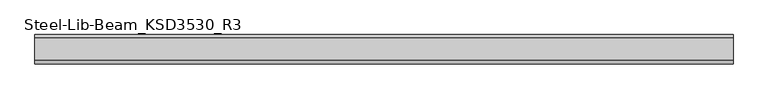
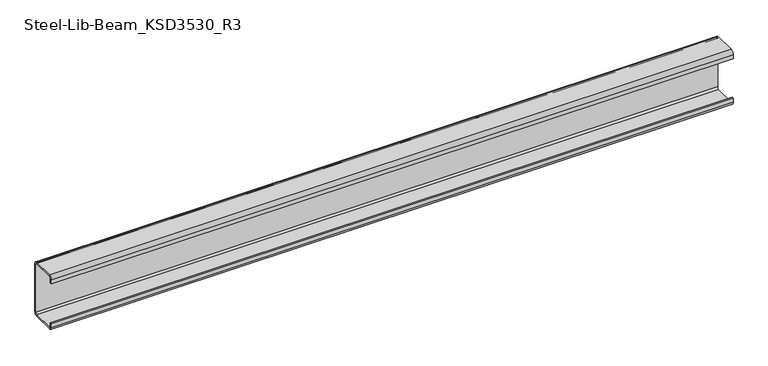
"""IFC4 building model written with IfcOpenShell, lengths in millimetres: beam geometry, Steel-Lib-Beam_KSD3530_R3 : BMS291_C-150×75x20x4.5."""

import ifcopenshell
import ifcopenshell.guid

model = None  # the IFC model being written
_history = None  # IfcOwnerHistory: only IFC2X3 demands one
_inside = {}  # id of a spatial element -> (the spatial element, [elements in it])
_under = {}  # id of a project, library or spatial element -> (it, [spatial elements below it])
_declared = {}  # id of a project -> (the project, [libraries it declares])
_typed = {}  # id of a type object -> (the type object, [elements of that type])
_made_of = {}  # id of a material, layer set ... -> (it, [elements and type objects made of it])


def new_model(schema):
    """Start an empty IFC model of exactly this schema.

    Asked for "IFC4X3", IfcOpenShell would pick the latest addendum, in which some entities
    have other attributes; the version numbers below select the first issue.
    IFC2X3 requires an IfcOwnerHistory on every rooted entity: one is made here for all.
    """
    global model, _history
    if schema == "IFC4X3":
        model = ifcopenshell.file(schema_version=(4, 3, 0, 0))
    else:
        model = ifcopenshell.file(schema=schema)
    _inside.clear()
    _under.clear()
    _declared.clear()
    _typed.clear()
    _made_of.clear()
    _history = None
    if model.schema == "IFC2X3":
        org = make("IfcOrganization", Name="unknown")
        user = make(
            "IfcPersonAndOrganization",
            ThePerson=make("IfcPerson", FamilyName="unknown"),
            TheOrganization=org,
        )
        app = make(
            "IfcApplication",
            ApplicationDeveloper=org,
            Version="unknown",
            ApplicationFullName="unknown",
            ApplicationIdentifier="unknown",
        )
        _history = make(
            "IfcOwnerHistory",
            OwningUser=user,
            OwningApplication=app,
            ChangeAction="ADDED",
            CreationDate=0,
        )
    return model


def make(cls, **values):
    """One entity of the class cls with the attributes given. An attribute that is None is left unset."""
    return model.create_entity(
        cls, **{name: value for name, value in values.items() if value is not None}
    )


def rooted(cls, **values):
    """An entity with a GlobalId (a new one), such as an element, a storey or a relation."""
    return make(cls, GlobalId=ifcopenshell.guid.new(), OwnerHistory=_history, **values)


def si_unit(unit_type, name, prefix=None):
    """IfcSIUnit, for example si_unit("LENGTHUNIT", "METRE", prefix="MILLI")."""
    return make("IfcSIUnit", UnitType=unit_type, Prefix=prefix, Name=name)


def assignment(units):
    """IfcUnitAssignment: the units of a project."""
    return None if units is None else make("IfcUnitAssignment", Units=units)


def point(xyz):
    """IfcCartesianPoint."""
    return None if xyz is None else make("IfcCartesianPoint", Coordinates=xyz)


def direction(xyz):
    """IfcDirection."""
    return None if xyz is None else make("IfcDirection", DirectionRatios=xyz)


def frame(location, z_axis=None, x_axis=None):
    """IfcAxis2Placement3D, a coordinate frame: its origin and axes. An axis left out is left unset."""
    return make(
        "IfcAxis2Placement3D",
        Location=point(location),
        Axis=direction(z_axis),
        RefDirection=direction(x_axis),
    )


def frame_2d(location, x_axis=None):
    """IfcAxis2Placement2D, a coordinate frame in the plane: its origin and x axis."""
    return make(
        "IfcAxis2Placement2D", Location=point(location), RefDirection=direction(x_axis)
    )


def origin():
    """The frame at (0, 0, 0) with its axes left unset."""
    return frame((0.0, 0.0, 0.0))


def place(relative_to, where):
    """IfcLocalPlacement: puts the frame where relative to a parent placement (None: the world)."""
    return make(
        "IfcLocalPlacement", PlacementRelTo=relative_to, RelativePlacement=where
    )


def context(
    kind, dimensions, precision=None, world=None, true_north=None, identifier=None
):
    """IfcGeometricRepresentationContext, for example the 3D "Model" context."""
    return make(
        "IfcGeometricRepresentationContext",
        ContextIdentifier=identifier,
        ContextType=kind,
        CoordinateSpaceDimension=dimensions,
        Precision=precision,
        WorldCoordinateSystem=world,
        TrueNorth=true_north,
    )


def project(units=None, contexts=None):
    """IfcProject with its units and contexts."""
    return rooted(
        "IfcProject",
        Name="project",
        RepresentationContexts=contexts,
        UnitsInContext=assignment(units),
    )


def spatial(cls, under=None, at=None, **own):
    """A site, building, storey or space (cls), placed at a placement, below another one or the project."""
    s = rooted(cls, ObjectPlacement=at, **own)
    if under is not None:
        _under.setdefault(under.id(), (under, []))[1].append(s)
    return s


def polyline(points):
    """IfcPolyline through the points."""
    return make("IfcPolyline", Points=[point(p) for p in points])


def circle_curve(where, radius):
    """IfcCircle in the frame where."""
    return make("IfcCircle", Position=where, Radius=radius)


def trimmed(basis, trim1, trim2, sense, master):
    """IfcTrimmedCurve: the piece of a basis curve between two trims."""
    return make(
        "IfcTrimmedCurve",
        BasisCurve=basis,
        Trim1=trim1,
        Trim2=trim2,
        SenseAgreement=sense,
        MasterRepresentation=master,
    )


def segment(curve, same_sense, transition):
    """IfcCompositeCurveSegment."""
    return make(
        "IfcCompositeCurveSegment",
        Transition=transition,
        SameSense=same_sense,
        ParentCurve=curve,
    )


def composite_curve(segments, self_intersect=None):
    """IfcCompositeCurve: segments joined end to end."""
    return make("IfcCompositeCurve", Segments=segments, SelfIntersect=self_intersect)


def outline(outer, holes=None, kind="AREA"):
    """IfcArbitraryClosedProfileDef: a profile drawn as a closed curve; with holes, ...WithVoids."""
    if holes is None:
        return make("IfcArbitraryClosedProfileDef", ProfileType=kind, OuterCurve=outer)
    return make(
        "IfcArbitraryProfileDefWithVoids",
        ProfileType=kind,
        OuterCurve=outer,
        InnerCurves=holes,
    )


def extrude(swept, where, along, depth):
    """IfcExtrudedAreaSolid: the profile swept, set in the frame where, extruded along a direction by depth."""
    return make(
        "IfcExtrudedAreaSolid",
        SweptArea=swept,
        Position=where,
        ExtrudedDirection=direction(along),
        Depth=depth,
    )


def shape(context_of_items, identifier, shape_type, items):
    """IfcShapeRepresentation: the items that make up one representation, for example the "Body"."""
    return make(
        "IfcShapeRepresentation",
        ContextOfItems=context_of_items,
        RepresentationIdentifier=identifier,
        RepresentationType=shape_type,
        Items=items,
    )


def source(mapping_origin, context_of_items, identifier, shape_type, items):
    """IfcRepresentationMap: a shape defined once, which mapped items show again and again."""
    return make(
        "IfcRepresentationMap",
        MappingOrigin=mapping_origin,
        MappedRepresentation=shape(context_of_items, identifier, shape_type, items),
    )


def transform(
    local_origin,
    x_axis=None,
    y_axis=None,
    z_axis=None,
    scale=None,
    scale2=None,
    scale3=None,
    uniform=True,
):
    """IfcCartesianTransformationOperator3D, or its non-uniform kind. x_axis, y_axis, z_axis: its Axis1, 2, 3."""
    if uniform:
        return make(
            "IfcCartesianTransformationOperator3D",
            Axis1=direction(x_axis),
            Axis2=direction(y_axis),
            LocalOrigin=point(local_origin),
            Scale=scale,
            Axis3=direction(z_axis),
        )
    return make(
        "IfcCartesianTransformationOperator3DnonUniform",
        Axis1=direction(x_axis),
        Axis2=direction(y_axis),
        LocalOrigin=point(local_origin),
        Scale=scale,
        Axis3=direction(z_axis),
        Scale2=scale2,
        Scale3=scale3,
    )


def mapped(mapping_source, mapping_target):
    """IfcMappedItem: shows the shape of a source again, moved by a transform."""
    return make(
        "IfcMappedItem", MappingSource=mapping_source, MappingTarget=mapping_target
    )


def made_of(thing, what):
    """Note that an element or type object is made of a material, layer set ...; save() writes the relation."""
    if what is not None:
        _made_of.setdefault(what.id(), (what, []))[1].append(thing)
    return thing


def element(
    cls,
    number,
    at=None,
    inside=None,
    cuts=None,
    type_object=None,
    material=None,
    context=None,
    identifier="Body",
    shape_type=None,
    held_by="IfcProductDefinitionShape",
    body=None,
    shapes=None,
    **own,
):
    """One element of the class cls, such as IfcWall. Its Tag is "e" and its number.

    at: its placement. inside: the storey or other place that contains it. cuts: it is an
    opening in that element (IfcRelVoidsElement). A single representation is given by context,
    identifier, shape_type and body (its items); several are given by shapes. held_by: the class
    of the entity that holds the representations. save() writes the other relations.
    """
    e = rooted(cls, Tag="e%d" % number, ObjectPlacement=at, **own)
    if body is not None:
        shapes = [shape(context, identifier, shape_type, body)]
    if shapes is not None:
        e.Representation = make(held_by, Representations=shapes)
    if inside is not None:
        _inside.setdefault(inside.id(), (inside, []))[1].append(e)
    if cuts is not None:
        rooted(
            "IfcRelVoidsElement", RelatingBuildingElement=cuts, RelatedOpeningElement=e
        )
    if type_object is not None:
        _typed.setdefault(type_object.id(), (type_object, []))[1].append(e)
    return made_of(e, material)


def aggregate(whole, parts):
    """IfcRelAggregates: a whole, such as a stair, and the parts it consists of."""
    return rooted("IfcRelAggregates", RelatingObject=whole, RelatedObjects=parts)


def save(model, path):
    """Write the relations noted so far, then the file.

    IfcRelAggregates (storeys below a building ...), IfcRelContainedInSpatialStructure (elements
    in a storey), IfcRelDefinesByType, IfcRelAssociatesMaterial and IfcRelDeclares: one each for
    every whole, place, type object, material and project.
    """
    for whole, parts in _under.values():
        aggregate(whole, parts)
    for where, things in _inside.values():
        rooted(
            "IfcRelContainedInSpatialStructure",
            RelatedElements=things,
            RelatingStructure=where,
        )
    for kind, things in _typed.values():
        rooted("IfcRelDefinesByType", RelatedObjects=things, RelatingType=kind)
    for what, things in _made_of.values():
        rooted("IfcRelAssociatesMaterial", RelatedObjects=things, RelatingMaterial=what)
    for by, libraries in _declared.values():
        rooted("IfcRelDeclares", RelatingContext=by, RelatedDefinitions=libraries)
    model.write(path)


def steel_lib_beam_ksd3530_r3_7e2e8e32(model_context):
    return source(origin(), model_context, "Body", "SweptSolid", [
        extrude(outline(composite_curve([segment(trimmed(circle_curve(frame_2d((-41.0, 66.0)), 9.0), [point((-50.0, 66.0))], [point((-41.0, 75.0))], False, "CARTESIAN"), True, "CONTINUOUS"), segment(polyline([(-41.0, 75.0), (16.0, 75.0)]), True, "CONTINUOUS"), segment(trimmed(circle_curve(frame_2d((16.0, 66.0)), 9.0), [point((16.0, 75.0))], [point((25.0, 66.0))], False, "CARTESIAN"), True, "CONTINUOUS"), segment(polyline([(25.0, 66.0), (25.0, -66.0)]), True, "CONTINUOUS"), segment(trimmed(circle_curve(frame_2d((16.0, -66.0)), 9.0), [point((25.0, -66.0))], [point((16.0, -75.0))], False, "CARTESIAN"), True, "CONTINUOUS"), segment(polyline([(16.0, -75.0), (-41.0, -75.0)]), True, "CONTINUOUS"), segment(trimmed(circle_curve(frame_2d((-41.0, -66.0)), 9.0), [point((-41.0, -75.0))], [point((-50.0, -66.0))], False, "CARTESIAN"), True, "CONTINUOUS"), segment(polyline([(-50.0, -66.0), (-50.0, -55.0), (-45.5, -55.0), (-45.5, -66.0)]), True, "CONTINUOUS"), segment(trimmed(circle_curve(frame_2d((-41.0, -66.0)), 4.5), [point((-45.5, -66.0))], [point((-41.0, -70.5))], True, "CARTESIAN"), True, "CONTINUOUS"), segment(polyline([(-41.0, -70.5), (16.0, -70.5)]), True, "CONTINUOUS"), segment(trimmed(circle_curve(frame_2d((16.0, -66.0)), 4.5), [point((16.0, -70.5))], [point((20.5, -66.0))], True, "CARTESIAN"), True, "CONTINUOUS"), segment(polyline([(20.5, -66.0), (20.5, 66.0)]), True, "CONTINUOUS"), segment(trimmed(circle_curve(frame_2d((16.0, 66.0)), 4.5), [point((20.5, 66.0))], [point((16.0, 70.5))], True, "CARTESIAN"), True, "CONTINUOUS"), segment(polyline([(16.0, 70.5), (-41.0, 70.5)]), True, "CONTINUOUS"), segment(trimmed(circle_curve(frame_2d((-41.0, 66.0)), 4.5), [point((-41.0, 70.5))], [point((-45.5, 66.0))], True, "CARTESIAN"), True, "CONTINUOUS"), segment(polyline([(-45.5, 66.0), (-45.5, 55.0), (-50.0, 55.0), (-50.0, 66.0)]), True, "CONTINUOUS")], self_intersect=False)), frame((-890.0, 0.0, 0.0), z_axis=(1.0, 0.0, 0.0), x_axis=(0.0, 1.0, 0.0)), (0.0, 0.0, 1.0), 1780.0),
    ])


if __name__ == "__main__":
    model = new_model("IFC4")
    model_context = context("Model", 3, world=origin())
    ifc_project = project(units=[si_unit("LENGTHUNIT", "METRE", prefix="MILLI")], contexts=[model_context])
    site = spatial("IfcSite", under=ifc_project)
    building = spatial("IfcBuilding", under=site)
    placement = place(None, origin())
    steel_lib_beam_ksd3530_r3_shape = steel_lib_beam_ksd3530_r3_7e2e8e32(model_context)
    element("IfcBeam", 1, ObjectType="Steel-Lib-Beam_KSD3530_R3 : BMS291_C-150×75x20x4.5", at=placement, inside=building, context=model_context, shape_type="MappedRepresentation", body=[
        mapped(steel_lib_beam_ksd3530_r3_shape, transform((0.0, 0.0, 0.0), x_axis=(1.0, 0.0, 0.0), y_axis=(0.0, 1.0, 0.0), z_axis=(0.0, 0.0, 1.0))),
    ])
    save(model, "model.ifc")

# Revit data of these elements
# Type "Steel-Lib-Beam_KSD3530_R3 : BMS291_C-150×75x20x4.5"
#   Keynote = "C-150×75x20x4.5"
#   SteelWeight = "Light"
#   x = 0.0250 m
#   t1 = 0.0090 m
#   t = 0.0045 m
#   Surface Area = 0.629834 m²/m
#   Section Area = 13.9688 cm²
#   Mass per Unit Length = 10.9655 kg/m
#   C = 0.0200 m
#   A = 0.0750 m
#   Length [instance default] = 1.5000 m
#   H = 0.1500 m
#   hec_material4 [instance default] = none
#   hec_material3 [instance default] = none
#   hec_material2 [instance default] = none
#   hec_material1 [instance default] = none
#   Structural Material [instance default] = Metal - Steel - Light Gauge
#   Assembly Code = ""
# Element 1 (IfcBeam, "Steel-Lib-Beam_KSD3530_R3 : BMS291_C-150×75x20x4.5")
#   Structural Material = none
# Materials
#   "Metal - Steel - Light Gauge": class "Metal", colour RGB 247 247 247, transparency 0
